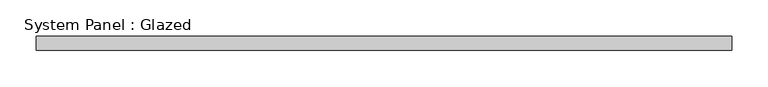
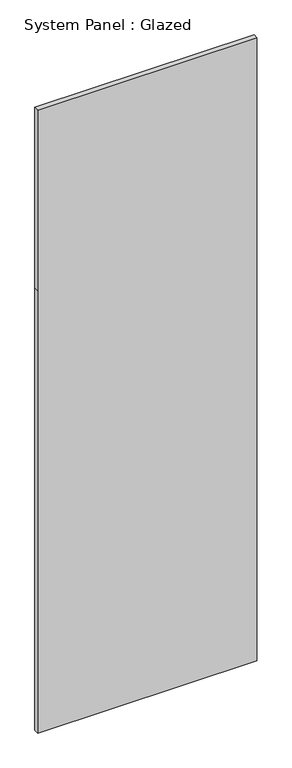
"""IFC4 building model written with IfcOpenShell, lengths in millimetres: plate geometry, System Panel : Glazed."""

from ifc_helpers import new_model, si_unit, frame, origin, place, context, project, spatial, polyline, outline, extrude, source, transform, mapped, element, save


def system_panel_glazed_3ea8b645(model_context):
    return source(origin(), model_context, "Body", "SweptSolid", [
        extrude(outline(polyline([(0.0, -482.5), (0.0, 482.5), (2060.0, 482.5), (2900.0, 482.5), (2900.0, -482.5), (2060.0, -482.5), (0.0, -482.5)])), frame((0.0, 0.0, 0.0), z_axis=(0.0, 1.0, 0.0), x_axis=(0.0, 0.0, 1.0)), (0.0, 0.0, 1.0), 20.0),
    ])


if __name__ == "__main__":
    model = new_model("IFC4")
    model_context = context("Model", 3, world=origin())
    ifc_project = project(units=[si_unit("LENGTHUNIT", "METRE", prefix="MILLI")], contexts=[model_context])
    site = spatial("IfcSite", under=ifc_project)
    building = spatial("IfcBuilding", under=site)
    placement = place(None, origin())
    system_panel_glazed_shape = system_panel_glazed_3ea8b645(model_context)
    element("IfcPlate", 1, ObjectType="System Panel : Glazed", at=placement, inside=building, context=model_context, shape_type="MappedRepresentation", body=[
        mapped(system_panel_glazed_shape, transform((0.0, 0.0, 0.0), x_axis=(1.0, 0.0, 0.0), y_axis=(0.0, 1.0, 0.0), z_axis=(0.0, 0.0, 1.0))),
    ])
    save(model, "model.ifc")

# Revit data of these elements
# Type "System Panel : Glazed"
#   COBie.Type = no
# Element 1 (IfcPlate, "System Panel : Glazed")
#   Materials on its faces: "Glass"
# Materials
#   "Glass": class "Glass", colour RGB 0 128 192, transparency 0.75, Description = "Soda Lime Glass", Cost = 0
